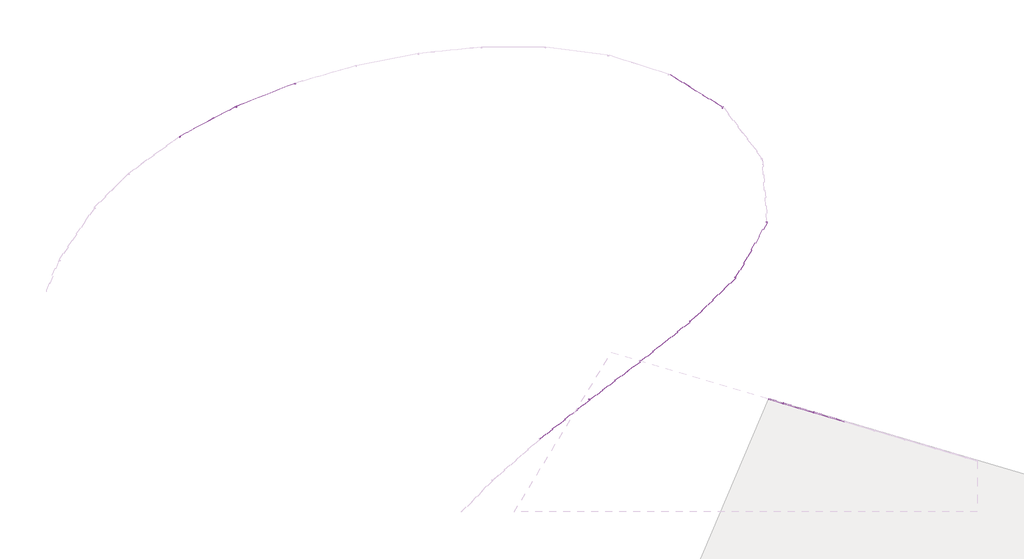
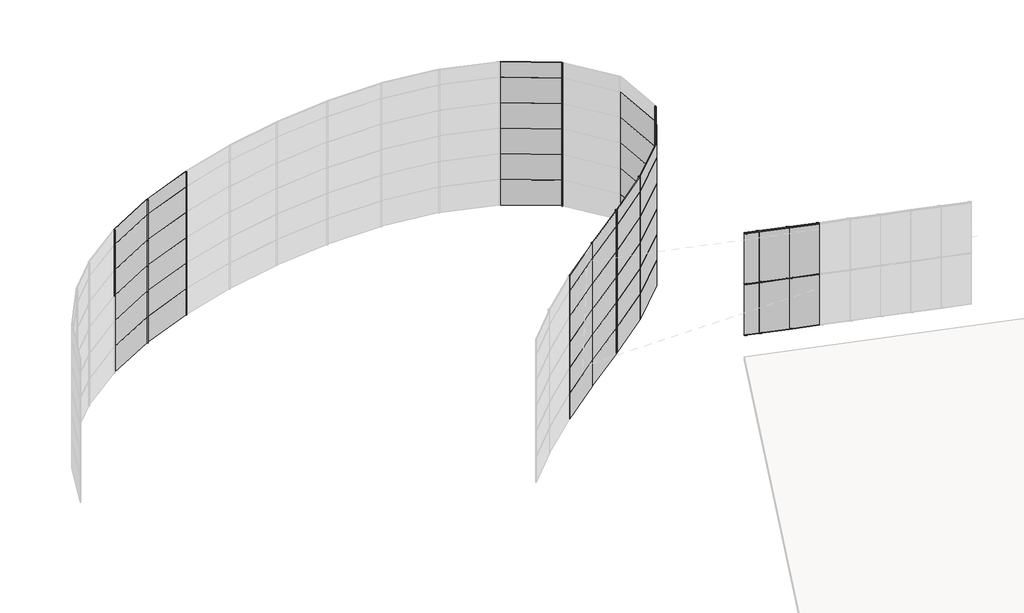
# One storey, part 6 of 8: 60 members, 59 plates.
# Revit data of these elements (continued)
# Type "Montante circular : 25 mm Raio"
#   built-in parameter 1007350 = 0.082021 (stored number, unit not read)
# Type "Painel do sistema : Envidraçado"
#   Construction Type Id = "GSP4R"
#   Analytic Construction = "Vidraça única Pilkington 1/8 pol"
#   Visual Light Transmittance = 0.9
#   Solar Heat Gain Coefficient = 0.86
#   Heat Transfer Coefficient (U) = 6.7069 W/(m²·K)
# Elements 1, 2, 3, 4, 5, 6, 7, 8, 9, 10, 11, 12, 13, 14, 15, 16, 17, 18, 19, 20, 21, 22, 23, 24, 25, 26, 27, 28, 29, 30, 31, 32, 33, 34, 35, 36, 37, 38, 39, 40, 41, 42, 43, 44, 45, 46, 47, 48, 49, 50, 51, 52, 53, 54, 55, 56, 57, 58, 59, 60 (IfcMember, "Montante circular : 25 mm Raio")
#   Phase Created = Construção nova
#   Materials on its faces: "Alumín."
# Elements 61, 62, 63, 64, 65, 66, 67, 68, 69, 70, 71, 72, 73, 74, 75, 76, 77, 78, 79, 80, 81, 82, 83, 84, 85, 86, 87, 88, 89, 90, 91, 92, 93, 94, 95, 96, 97, 98, 99, 100, 101, 102, 103, 104, 105, 106, 107, 108, 109, 110, 111, 112, 113, 114, 115, 116, 117, 118, 119 (IfcPlate, "Painel do sistema : Envidraçado")
#   Phase Created = Construção nova
#   Materials on its faces: "Vidro"
# Materials
#   "Alumín.": class "Metal", colour RGB 247 247 247, transparency 0, Description = "Alumín. 6061", Cost = 0
#   "Vidro": class "Vidro", colour RGB 0 128 192, transparency 0.9, Description = "Vidro de sílica", Cost = 0
